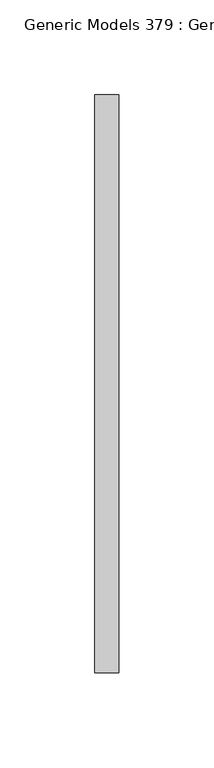
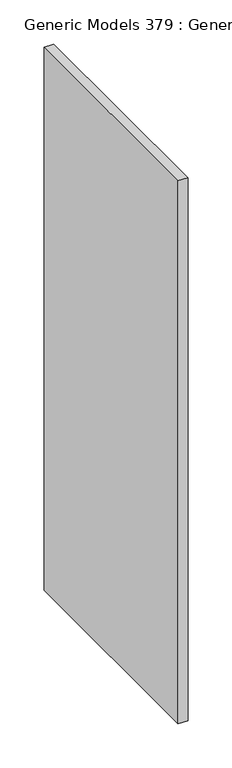
"""IFC4 building model written with IfcOpenShell, lengths in millimetres: proxy geometry, Generic Models 379 : Generic Models 349."""

from ifc_helpers import new_model, si_unit, frame, origin, place, context, project, spatial, polyline, outline, extrude, source, transform, mapped, element, save


def generic_models_379_generic_models_349_d90945c3(model_context):
    return source(origin(), model_context, "Body", "SweptSolid", [
        extrude(outline(polyline([(-6439.0736296, -4250.542257), (-6451.7736295, -4250.542257), (-6451.7736295, -3945.742257), (-6439.0736296, -3945.742257), (-6439.0736296, -4250.542257)])), frame((0.0, 0.0, 126641.6834738), z_axis=(0.0, 0.0, 1.0), x_axis=(1.0, 0.0, 0.0)), (0.0, 0.0, 1.0), 752.2945112),
    ])


if __name__ == "__main__":
    model = new_model("IFC4")
    model_context = context("Model", 3, world=origin())
    ifc_project = project(units=[si_unit("LENGTHUNIT", "METRE", prefix="MILLI")], contexts=[model_context])
    site = spatial("IfcSite", under=ifc_project)
    building = spatial("IfcBuilding", under=site)
    placement = place(None, origin())
    generic_models_379_generic_models_349_shape = generic_models_379_generic_models_349_d90945c3(model_context)
    element("IfcBuildingElementProxy", 1, Name="Generic Models 379 : Generic Models 349", ObjectType="Generic Models 379 : Generic Models 349", at=placement, inside=building, context=model_context, shape_type="MappedRepresentation", body=[
        mapped(generic_models_379_generic_models_349_shape, transform((0.0, 0.0, 0.0), x_axis=(1.0, 0.0, 0.0), y_axis=(0.0, 1.0, 0.0), z_axis=(0.0, 0.0, 1.0))),
    ])
    save(model, "model.ifc")

# Revit data of these elements
# Element 1 (IfcBuildingElementProxy, "Generic Models 379 : Generic Models 349")
#   Materials on its faces: "_5/8\" DRYWALL"
# Materials
#   "_5/8\" DRYWALL": class "Generic", colour RGB 191 191 191, transparency 0, Cost = 0
